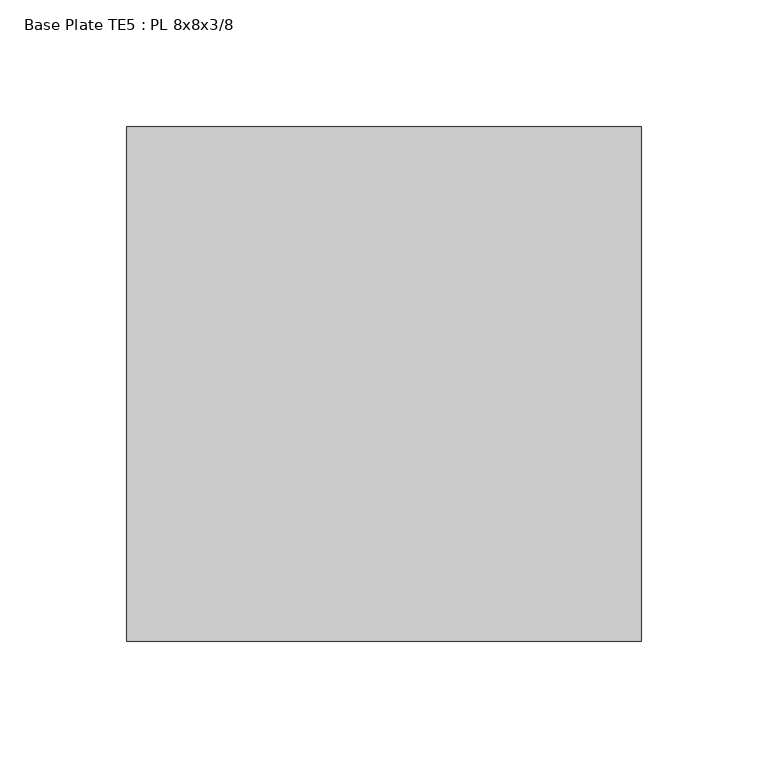
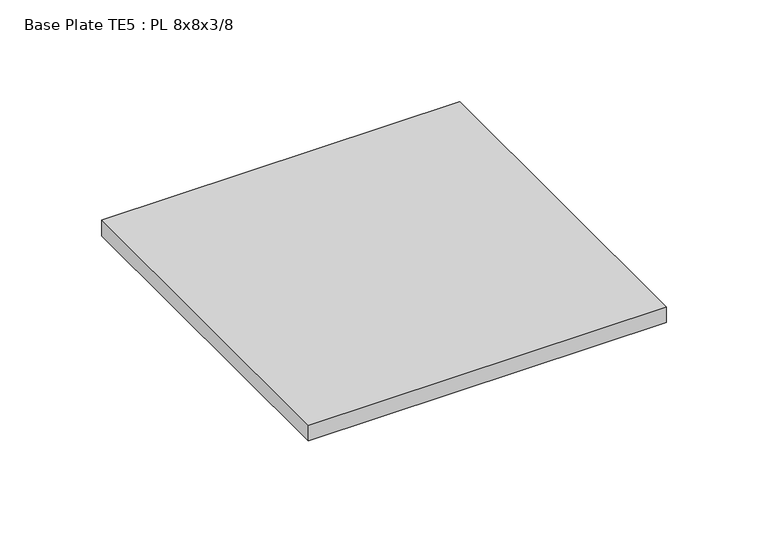
"""IFC4 building model written with IfcOpenShell, lengths in millimetres: proxy geometry, Base Plate TE5 : PL 8x8x3/8."""

from ifc_helpers import new_model, si_unit, frame, origin, place, context, project, spatial, polyline, outline, extrude, source, transform, mapped, element, save


def base_plate_te5_pl_8x8x3_8_4141263b(model_context):
    return source(origin(), model_context, "Body", "SweptSolid", [
        extrude(outline(polyline([(587365.8770246, -536468.3913841), (587365.8770246, -536265.1913841), (587569.0770246, -536265.1913841), (587569.0770246, -536468.3913841), (587365.8770246, -536468.3913841)])), frame((0.0, 0.0, 19.05), z_axis=(0.0, 0.0, 1.0), x_axis=(1.0, 0.0, 0.0)), (0.0, 0.0, 1.0), 9.525),
    ])


if __name__ == "__main__":
    model = new_model("IFC4")
    model_context = context("Model", 3, world=origin())
    ifc_project = project(units=[si_unit("LENGTHUNIT", "METRE", prefix="MILLI")], contexts=[model_context])
    site = spatial("IfcSite", under=ifc_project)
    building = spatial("IfcBuilding", under=site)
    placement = place(None, origin())
    base_plate_te5_pl_8x8x3_8_shape = base_plate_te5_pl_8x8x3_8_4141263b(model_context)
    element("IfcBuildingElementProxy", 1, Name="Base Plate TE5 : PL 8x8x3/8", ObjectType="Base Plate TE5 : PL 8x8x3/8", at=placement, inside=building, context=model_context, shape_type="MappedRepresentation", body=[
        mapped(base_plate_te5_pl_8x8x3_8_shape, transform((0.0, 0.0, 0.0), x_axis=(1.0, 0.0, 0.0), y_axis=(0.0, 1.0, 0.0), z_axis=(0.0, 0.0, 1.0))),
    ])
    save(model, "model.ifc")

# Revit data of these elements
# Element 1 (IfcBuildingElementProxy, "Base Plate TE5 : PL 8x8x3/8")
#   Materials on its faces: "GALV. STL BASE PLATE"
# Materials
#   "GALV. STL BASE PLATE": class "Generic", colour RGB 211 211 207, transparency 0, Cost = 0
